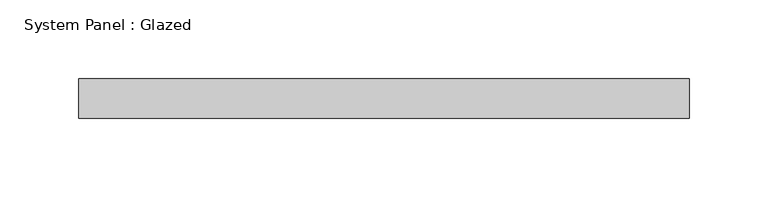
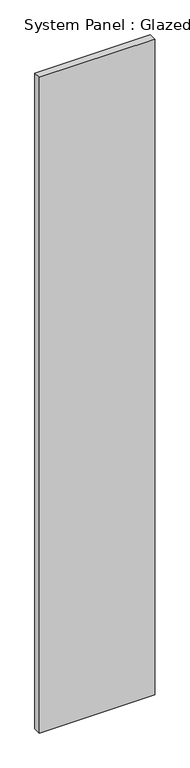
"""IFC4 building model written with IfcOpenShell, lengths in millimetres: plate geometry, System Panel : Glazed."""

from ifc_helpers import new_model, si_unit, origin, origin_with_axes, place, context, project, spatial, polyline, outline, extrude, source, transform, mapped, element, save


def system_panel_glazed_90de7002(model_context):
    return source(origin(), model_context, "Body", "SweptSolid", [
        extrude(outline(polyline([(193.75, 24.5), (-193.75, 24.5), (-193.75, 49.5), (193.75, 49.5), (193.75, 24.5)])), origin_with_axes(), (0.0, 0.0, 1.0), 2325.0),
    ])


if __name__ == "__main__":
    model = new_model("IFC4")
    model_context = context("Model", 3, world=origin())
    ifc_project = project(units=[si_unit("LENGTHUNIT", "METRE", prefix="MILLI")], contexts=[model_context])
    site = spatial("IfcSite", under=ifc_project)
    building = spatial("IfcBuilding", under=site)
    placement = place(None, origin())
    system_panel_glazed_shape = system_panel_glazed_90de7002(model_context)
    element("IfcPlate", 1, ObjectType="System Panel : Glazed", at=placement, inside=building, context=model_context, shape_type="MappedRepresentation", body=[
        mapped(system_panel_glazed_shape, transform((0.0, 0.0, 0.0), x_axis=(1.0, 0.0, 0.0), y_axis=(0.0, 1.0, 0.0), z_axis=(0.0, 0.0, 1.0))),
    ])
    save(model, "model.ifc")

# Revit data of these elements
# Type "System Panel : Glazed"
#   Construction Type Id = "GSP4R"
#   Analytic Construction = "1/8 in Pilkington single glazing"
#   Visual Light Transmittance = 0.9
#   Solar Heat Gain Coefficient = 0.86
#   Heat Transfer Coefficient (U) = 6.7069 W/(m²·K)
#   Define Thermal Properties by = 1
# Element 1 (IfcPlate, "System Panel : Glazed")
#   Materials on its faces: "Glass"
# Materials
#   "Glass": class "Glass", colour RGB 0 128 192, transparency 0.9, Description = "Soda Lime Glass", Cost = 0
